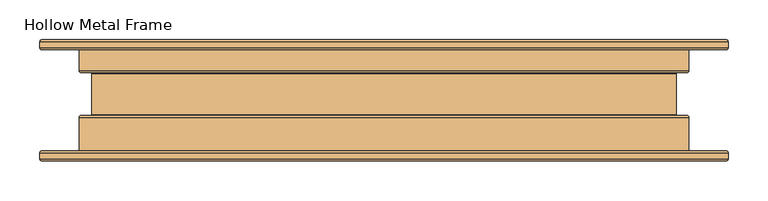
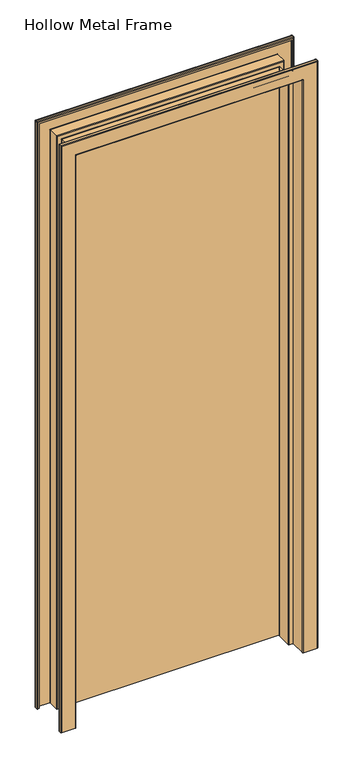
"""IFC4 building model written with IfcOpenShell, lengths in millimetres: door geometry, Hollow Metal Frame."""

from ifc_helpers import new_model, si_unit, frame, origin, origin_with_axes, place, context, project, spatial, polyline, circle_curve, ellipse_curve, outline, extrude, source, transform, mapped, element, save
from ifc_brep_helpers import plane_surface, cylinder_surface, revolved_surface, advanced_brep


def hollow_metal_frame_84e10a40(model_context):
    return source(origin(), model_context, "Body", "SolidModel", [
        advanced_brep(
        [(-429.22825, -63.5635, 0.0), (-423.8625, -63.5635, 0.0), (-423.8625, -65.11925, 0.0), (-429.22825, -65.11925, 0.0), (-430.24425, -66.13525, 0.0), (-430.24425, -73.66, 0.0), (-429.22825, -74.676, 0.0), (-383.57175, -74.676, 0.0), (-382.55575, -73.66, 0.0), (-382.55575, -21.68525, 0.0), (-379.984, -19.1135, 0.0), (-367.69675, -19.1135, 0.0), (-366.68075, -18.0975, 0.0), (-366.68075, 33.6931, 0.0), (-367.69675, 34.7091, 0.0), (-379.984, 34.7091, 0.0), (-382.55575, 37.28085, 0.0), (-382.55575, 73.5965, 0.0), (-383.57175, 74.6125, 0.0), (-429.22825, 74.6125, 0.0), (-430.24425, 73.5965, 0.0), (-430.24425, 66.07175, 0.0), (-429.22825, 65.05575, 0.0), (-423.8625, 65.05575, 0.0), (-423.8625, 63.5, 0.0), (-429.22825, 63.5, 0.0), (-431.8, 66.07175, 0.0), (-431.8, 73.5965, 0.0), (-429.22825, 76.16825, 0.0), (-383.57175, 76.16825, 0.0), (-381.0, 73.5965, 0.0), (-381.0, 37.28085, 0.0), (-379.984, 36.26485, 0.0), (-367.69675, 36.26485, 0.0), (-365.125, 33.6931, 0.0), (-365.125, -18.0975, 0.0), (-367.69675, -20.66925, 0.0), (-379.984, -20.66925, 0.0), (-381.0, -21.68525, 0.0), (-381.0, -73.66, 0.0), (-383.57175, -76.23175, 0.0), (-429.22825, -76.23175, 0.0), (-431.8, -73.66, 0.0), (-431.8, -66.13525, 0.0), (-431.8, -66.13525, 2082.8000001), (-429.22825, -63.5635, 2080.2282501), (-431.8, -73.66, 2082.8000001), (-429.22825, -76.23175, 2080.2282501), (-383.57175, -76.23175, 2034.5717501), (383.57175, -76.23175, 2034.5717501), (383.57175, -76.23175, 0.0), (429.22825, -76.23175, 0.0), (429.22825, -76.23175, 2080.2282501), (-381.0, -73.66, 2032.0000001), (-381.0, -21.68525, 2032.0000001), (-379.984, -20.66925, 2030.9840001), (-367.69675, -20.66925, 2018.6967501), (367.69675, -20.66925, 2018.6967501), (367.69675, -20.66925, 0.0), (379.984, -20.66925, 0.0), (379.984, -20.66925, 2030.9840001), (-365.125, -18.0975, 2016.1250001), (-365.125, 33.6931, 2016.1250001), (-367.69675, 36.26485, 2018.6967501), (-379.984, 36.26485, 2030.9840001), (379.984, 36.26485, 2030.9840001), (379.984, 36.26485, 0.0), (367.69675, 36.26485, 0.0), (367.69675, 36.26485, 2018.6967501), (-381.0, 37.28085, 2032.0000001), (-381.0, 73.5965, 2032.0000001), (-383.57175, 76.16825, 2034.5717501), (-429.22825, 76.16825, 2080.2282501), (429.22825, 76.16825, 2080.2282501), (429.22825, 76.16825, 0.0), (383.57175, 76.16825, 0.0), (383.57175, 76.16825, 2034.5717501), (-431.8, 73.5965, 2082.8000001), (-431.8, 66.07175, 2082.8000001), (-429.22825, 63.5, 2080.2282501), (-423.8625, 63.5, 2074.8625001), (423.8625, 63.5, 2074.8625001), (423.8625, 63.5, 0.0), (429.22825, 63.5, 0.0), (429.22825, 63.5, 2080.2282501), (-423.8625, 65.05575, 2074.8625001), (-429.22825, 65.05575, 2080.2282501), (429.22825, 65.05575, 2080.2282501), (429.22825, 65.05575, 0.0), (423.8625, 65.05575, 0.0), (423.8625, 65.05575, 2074.8625001), (-430.24425, 66.07175, 2081.2442501), (-430.24425, 73.5965, 2081.2442501), (-429.22825, 74.6125, 2080.2282501), (-383.57175, 74.6125, 2034.5717501), (383.57175, 74.6125, 2034.5717501), (383.57175, 74.6125, 0.0), (429.22825, 74.6125, 0.0), (429.22825, 74.6125, 2080.2282501), (-382.55575, 73.5965, 2033.5557501), (-382.55575, 37.28085, 2033.5557501), (-379.984, 34.7091, 2030.9840001), (-367.69675, 34.7091, 2018.6967501), (367.69675, 34.7091, 2018.6967501), (367.69675, 34.7091, 0.0), (379.984, 34.7091, 0.0), (379.984, 34.7091, 2030.9840001), (-366.68075, 33.6931, 2017.6807501), (-366.68075, -18.0975, 2017.6807501), (-367.69675, -19.1135, 2018.6967501), (-379.984, -19.1135, 2030.9840001), (379.984, -19.1135, 2030.9840001), (379.984, -19.1135, 0.0), (367.69675, -19.1135, 0.0), (367.69675, -19.1135, 2018.6967501), (-382.55575, -21.68525, 2033.5557501), (-382.55575, -73.66, 2033.5557501), (-383.57175, -74.676, 2034.5717501), (-429.22825, -74.676, 2080.2282501), (429.22825, -74.676, 2080.2282501), (429.22825, -74.676, 0.0), (383.57175, -74.676, 0.0), (383.57175, -74.676, 2034.5717501), (-430.24425, -73.66, 2081.2442501), (-430.24425, -66.13525, 2081.2442501), (-429.22825, -65.11925, 2080.2282501), (-423.8625, -65.11925, 2074.8625001), (423.8625, -65.11925, 2074.8625001), (423.8625, -65.11925, 0.0), (429.22825, -65.11925, 0.0), (429.22825, -65.11925, 2080.2282501), (-423.8625, -63.5635, 2074.8625001), (429.22825, -63.5635, 2080.2282501), (429.22825, -63.5635, 0.0), (423.8625, -63.5635, 0.0), (423.8625, -63.5635, 2074.8625001), (431.8, -66.13525, 2082.8000001), (431.8, -73.66, 2082.8000001), (381.0, -73.66, 2032.0000001), (381.0, -21.68525, 2032.0000001), (365.125, -18.0975, 2016.1250001), (365.125, 33.6931, 2016.1250001), (381.0, 37.28085, 2032.0000001), (381.0, 73.5965, 2032.0000001), (431.8, 73.5965, 2082.8000001), (431.8, 66.07175, 2082.8000001), (430.24425, 66.07175, 2081.2442501), (430.24425, 73.5965, 2081.2442501), (382.55575, 73.5965, 2033.5557501), (382.55575, 37.28085, 2033.5557501), (366.68075, 33.6931, 2017.6807501), (366.68075, -18.0975, 2017.6807501), (382.55575, -21.68525, 2033.5557501), (382.55575, -73.66, 2033.5557501), (430.24425, -73.66, 2081.2442501), (430.24425, -66.13525, 2081.2442501), (431.8, -66.13525, 0.0), (431.8, -73.66, 0.0), (381.0, -73.66, 0.0), (381.0, -21.68525, 0.0), (365.125, -18.0975, 0.0), (365.125, 33.6931, 0.0), (381.0, 37.28085, 0.0), (381.0, 73.5965, 0.0), (431.8, 73.5965, 0.0), (431.8, 66.07175, 0.0), (430.24425, 66.07175, 0.0), (430.24425, 73.5965, 0.0), (382.55575, 73.5965, 0.0), (382.55575, 37.28085, 0.0), (366.68075, 33.6931, 0.0), (366.68075, -18.0975, 0.0), (382.55575, -21.68525, 0.0), (382.55575, -73.66, 0.0), (430.24425, -73.66, 0.0), (430.24425, -66.13525, 0.0)],
        [
            (0, 1),
            (1, 2),
            (2, 3),
            (3, 4, circle_curve(frame((-429.22825, -66.13525, 0.0), z_axis=(0.0, 0.0, 1.0), x_axis=(0.0, 1.0, 0.0)), 1.016)),
            (4, 5),
            (5, 6, circle_curve(frame((-429.22825, -73.66, 0.0), z_axis=(0.0, 0.0, 1.0), x_axis=(0.0, 1.0, 0.0)), 1.016)),
            (6, 7),
            (7, 8, circle_curve(frame((-383.57175, -73.66, 0.0), z_axis=(0.0, 0.0, 1.0), x_axis=(0.0, 1.0, 0.0)), 1.016)),
            (8, 9),
            (9, 10, circle_curve(frame((-379.984, -21.68525, 0.0), z_axis=(0.0, 0.0, -1.0), x_axis=(0.0, 1.0, 0.0)), 2.57175)),
            (10, 11),
            (11, 12, circle_curve(frame((-367.69675, -18.0975, 0.0), z_axis=(0.0, 0.0, 1.0), x_axis=(0.0, 1.0, 0.0)), 1.016)),
            (12, 13),
            (13, 14, circle_curve(frame((-367.69675, 33.6931, 0.0), z_axis=(0.0, 0.0, 1.0), x_axis=(0.0, 1.0, 0.0)), 1.016)),
            (14, 15),
            (15, 16, circle_curve(frame((-379.984, 37.28085, 0.0), z_axis=(0.0, 0.0, -1.0), x_axis=(0.0, 1.0, 0.0)), 2.57175)),
            (16, 17),
            (17, 18, circle_curve(frame((-383.57175, 73.5965, 0.0), z_axis=(0.0, 0.0, 1.0), x_axis=(0.0, 1.0, 0.0)), 1.016)),
            (18, 19),
            (19, 20, circle_curve(frame((-429.22825, 73.5965, 0.0), z_axis=(0.0, 0.0, 1.0), x_axis=(0.0, 1.0, 0.0)), 1.016)),
            (20, 21),
            (21, 22, circle_curve(frame((-429.22825, 66.07175, 0.0), z_axis=(0.0, 0.0, 1.0), x_axis=(0.0, 1.0, 0.0)), 1.016)),
            (22, 23),
            (23, 24),
            (24, 25),
            (25, 26, circle_curve(frame((-429.22825, 66.07175, 0.0), z_axis=(0.0, 0.0, -1.0), x_axis=(0.0, 1.0, 0.0)), 2.57175)),
            (26, 27),
            (27, 28, circle_curve(frame((-429.22825, 73.5965, 0.0), z_axis=(0.0, 0.0, -1.0), x_axis=(0.0, 1.0, 0.0)), 2.57175)),
            (28, 29),
            (29, 30, circle_curve(frame((-383.57175, 73.5965, 0.0), z_axis=(0.0, 0.0, -1.0), x_axis=(0.0, 1.0, 0.0)), 2.57175)),
            (30, 31),
            (31, 32, circle_curve(frame((-379.984, 37.28085, 0.0), z_axis=(0.0, 0.0, 1.0), x_axis=(0.0, 1.0, 0.0)), 1.016)),
            (32, 33),
            (33, 34, circle_curve(frame((-367.69675, 33.6931, 0.0), z_axis=(0.0, 0.0, -1.0), x_axis=(0.0, 1.0, 0.0)), 2.57175)),
            (34, 35),
            (35, 36, circle_curve(frame((-367.69675, -18.0975, 0.0), z_axis=(0.0, 0.0, -1.0), x_axis=(0.0, 1.0, 0.0)), 2.57175)),
            (36, 37),
            (37, 38, circle_curve(frame((-379.984, -21.68525, 0.0), z_axis=(0.0, 0.0, 1.0), x_axis=(0.0, 1.0, 0.0)), 1.016)),
            (38, 39),
            (39, 40, circle_curve(frame((-383.57175, -73.66, 0.0), z_axis=(0.0, 0.0, -1.0), x_axis=(0.0, 1.0, 0.0)), 2.57175)),
            (40, 41),
            (41, 42, circle_curve(frame((-429.22825, -73.66, 0.0), z_axis=(0.0, 0.0, -1.0), x_axis=(0.0, 1.0, 0.0)), 2.57175)),
            (42, 43),
            (43, 0, circle_curve(frame((-429.22825, -66.13525, 0.0), z_axis=(0.0, 0.0, -1.0), x_axis=(0.0, 1.0, 0.0)), 2.57175)),
            (43, 44),
            (44, 45, ellipse_curve(frame((-429.22825, -66.13525, 2080.2282501), z_axis=(-0.7071067811865475, 0.0, -0.7071067811865475), x_axis=(0.7071067811865474, 0.0, -0.7071067811865476)), 3.6370037, 2.57175)),
            (45, 0),
            (42, 46),
            (46, 44),
            (41, 47),
            (47, 46, ellipse_curve(frame((-429.22825, -73.66, 2080.2282501), z_axis=(-0.7071067811865475, 0.0, -0.7071067811865475), x_axis=(0.7071067811865474, 0.0, -0.7071067811865476)), 3.6370037, 2.57175)),
            (40, 48),
            (48, 49),
            (49, 50),
            (50, 51),
            (51, 52),
            (52, 47),
            (39, 53),
            (53, 48, ellipse_curve(frame((-383.57175, -73.66, 2034.5717501), z_axis=(-0.7071067811865475, 0.0, -0.7071067811865475), x_axis=(0.7071067811865474, 0.0, -0.7071067811865476)), 3.6370037, 2.57175)),
            (38, 54),
            (54, 53),
            (37, 55),
            (55, 54, ellipse_curve(frame((-379.984, -21.68525, 2030.9840001), z_axis=(0.7071067811865475, 0.0, 0.7071067811865475), x_axis=(-0.7071067811865474, 0.0, 0.7071067811865476)), 1.436841, 1.016)),
            (36, 56),
            (56, 57),
            (57, 58),
            (58, 59),
            (59, 60),
            (60, 55),
            (35, 61),
            (61, 56, ellipse_curve(frame((-367.69675, -18.0975, 2018.6967501), z_axis=(-0.7071067811865475, 0.0, -0.7071067811865475), x_axis=(0.7071067811865474, 0.0, -0.7071067811865476)), 3.6370037, 2.57175)),
            (34, 62),
            (62, 61),
            (33, 63),
            (63, 62, ellipse_curve(frame((-367.69675, 33.6931, 2018.6967501), z_axis=(-0.7071067811865475, 0.0, -0.7071067811865475), x_axis=(0.7071067811865474, 0.0, -0.7071067811865476)), 3.6370037, 2.57175)),
            (32, 64),
            (64, 65),
            (65, 66),
            (66, 67),
            (67, 68),
            (68, 63),
            (31, 69),
            (69, 64, ellipse_curve(frame((-379.984, 37.28085, 2030.9840001), z_axis=(0.7071067811865475, 0.0, 0.7071067811865475), x_axis=(-0.7071067811865474, 0.0, 0.7071067811865476)), 1.436841, 1.016)),
            (30, 70),
            (70, 69),
            (29, 71),
            (71, 70, ellipse_curve(frame((-383.57175, 73.5965, 2034.5717501), z_axis=(-0.7071067811865475, 0.0, -0.7071067811865475), x_axis=(0.7071067811865474, 0.0, -0.7071067811865476)), 3.6370037, 2.57175)),
            (28, 72),
            (72, 73),
            (73, 74),
            (74, 75),
            (75, 76),
            (76, 71),
            (27, 77),
            (77, 72, ellipse_curve(frame((-429.22825, 73.5965, 2080.2282501), z_axis=(-0.7071067811865475, 0.0, -0.7071067811865475), x_axis=(0.7071067811865474, 0.0, -0.7071067811865476)), 3.6370037, 2.57175)),
            (26, 78),
            (78, 77),
            (25, 79),
            (79, 78, ellipse_curve(frame((-429.22825, 66.07175, 2080.2282501), z_axis=(-0.7071067811865475, 0.0, -0.7071067811865475), x_axis=(0.7071067811865474, 0.0, -0.7071067811865476)), 3.6370037, 2.57175)),
            (24, 80),
            (80, 81),
            (81, 82),
            (82, 83),
            (83, 84),
            (84, 79),
            (23, 85),
            (85, 80),
            (22, 86),
            (86, 87),
            (87, 88),
            (88, 89),
            (89, 90),
            (90, 85),
            (21, 91),
            (91, 86, ellipse_curve(frame((-429.22825, 66.07175, 2080.2282501), z_axis=(0.7071067811865475, 0.0, 0.7071067811865475), x_axis=(-0.7071067811865474, 0.0, 0.7071067811865476)), 1.436841, 1.016)),
            (20, 92),
            (92, 91),
            (19, 93),
            (93, 92, ellipse_curve(frame((-429.22825, 73.5965, 2080.2282501), z_axis=(0.7071067811865475, 0.0, 0.7071067811865475), x_axis=(-0.7071067811865474, 0.0, 0.7071067811865476)), 1.436841, 1.016)),
            (18, 94),
            (94, 95),
            (95, 96),
            (96, 97),
            (97, 98),
            (98, 93),
            (17, 99),
            (99, 94, ellipse_curve(frame((-383.57175, 73.5965, 2034.5717501), z_axis=(0.7071067811865475, 0.0, 0.7071067811865475), x_axis=(-0.7071067811865474, 0.0, 0.7071067811865476)), 1.436841, 1.016)),
            (16, 100),
            (100, 99),
            (15, 101),
            (101, 100, ellipse_curve(frame((-379.984, 37.28085, 2030.9840001), z_axis=(-0.7071067811865475, 0.0, -0.7071067811865475), x_axis=(0.7071067811865474, 0.0, -0.7071067811865476)), 3.6370037, 2.57175)),
            (14, 102),
            (102, 103),
            (103, 104),
            (104, 105),
            (105, 106),
            (106, 101),
            (13, 107),
            (107, 102, ellipse_curve(frame((-367.69675, 33.6931, 2018.6967501), z_axis=(0.7071067811865475, 0.0, 0.7071067811865475), x_axis=(-0.7071067811865474, 0.0, 0.7071067811865476)), 1.436841, 1.016)),
            (12, 108),
            (108, 107),
            (11, 109),
            (109, 108, ellipse_curve(frame((-367.69675, -18.0975, 2018.6967501), z_axis=(0.7071067811865475, 0.0, 0.7071067811865475), x_axis=(-0.7071067811865474, 0.0, 0.7071067811865476)), 1.436841, 1.016)),
            (10, 110),
            (110, 111),
            (111, 112),
            (112, 113),
            (113, 114),
            (114, 109),
            (9, 115),
            (115, 110, ellipse_curve(frame((-379.984, -21.68525, 2030.9840001), z_axis=(-0.7071067811865475, 0.0, -0.7071067811865475), x_axis=(0.7071067811865474, 0.0, -0.7071067811865476)), 3.6370037, 2.57175)),
            (8, 116),
            (116, 115),
            (7, 117),
            (117, 116, ellipse_curve(frame((-383.57175, -73.66, 2034.5717501), z_axis=(0.7071067811865475, 0.0, 0.7071067811865475), x_axis=(-0.7071067811865474, 0.0, 0.7071067811865476)), 1.436841, 1.016)),
            (6, 118),
            (118, 119),
            (119, 120),
            (120, 121),
            (121, 122),
            (122, 117),
            (5, 123),
            (123, 118, ellipse_curve(frame((-429.22825, -73.66, 2080.2282501), z_axis=(0.7071067811865475, 0.0, 0.7071067811865475), x_axis=(-0.7071067811865474, 0.0, 0.7071067811865476)), 1.436841, 1.016)),
            (4, 124),
            (124, 123),
            (3, 125),
            (125, 124, ellipse_curve(frame((-429.22825, -66.13525, 2080.2282501), z_axis=(0.7071067811865475, 0.0, 0.7071067811865475), x_axis=(-0.7071067811865474, 0.0, 0.7071067811865476)), 1.436841, 1.016)),
            (2, 126),
            (126, 127),
            (127, 128),
            (128, 129),
            (129, 130),
            (130, 125),
            (1, 131),
            (131, 126),
            (45, 132),
            (132, 133),
            (133, 134),
            (134, 135),
            (135, 131),
            (44, 136),
            (136, 132, ellipse_curve(frame((429.22825, -66.13525, 2080.2282501), z_axis=(-0.7071067811865475, 0.0, 0.7071067811865475), x_axis=(-0.7071067811865476, 0.0, -0.7071067811865474)), 3.6370037, 2.57175)),
            (46, 137),
            (137, 136),
            (52, 137, ellipse_curve(frame((429.22825, -73.66, 2080.2282501), z_axis=(-0.7071067811865475, 0.0, 0.7071067811865475), x_axis=(-0.7071067811865476, 0.0, -0.7071067811865474)), 3.6370037, 2.57175)),
            (53, 138),
            (138, 49, ellipse_curve(frame((383.57175, -73.66, 2034.5717501), z_axis=(-0.7071067811865475, 0.0, 0.7071067811865475), x_axis=(-0.7071067811865476, 0.0, -0.7071067811865474)), 3.6370037, 2.57175)),
            (54, 139),
            (139, 138),
            (60, 139, ellipse_curve(frame((379.984, -21.68525, 2030.9840001), z_axis=(0.7071067811865475, 0.0, -0.7071067811865475), x_axis=(0.7071067811865476, 0.0, 0.7071067811865474)), 1.436841, 1.016)),
            (61, 140),
            (140, 57, ellipse_curve(frame((367.69675, -18.0975, 2018.6967501), z_axis=(-0.7071067811865475, 0.0, 0.7071067811865475), x_axis=(-0.7071067811865476, 0.0, -0.7071067811865474)), 3.6370037, 2.57175)),
            (62, 141),
            (141, 140),
            (68, 141, ellipse_curve(frame((367.69675, 33.6931, 2018.6967501), z_axis=(-0.7071067811865475, 0.0, 0.7071067811865475), x_axis=(-0.7071067811865476, 0.0, -0.7071067811865474)), 3.6370037, 2.57175)),
            (69, 142),
            (142, 65, ellipse_curve(frame((379.984, 37.28085, 2030.9840001), z_axis=(0.7071067811865475, 0.0, -0.7071067811865475), x_axis=(0.7071067811865476, 0.0, 0.7071067811865474)), 1.436841, 1.016)),
            (70, 143),
            (143, 142),
            (76, 143, ellipse_curve(frame((383.57175, 73.5965, 2034.5717501), z_axis=(-0.7071067811865475, 0.0, 0.7071067811865475), x_axis=(-0.7071067811865476, 0.0, -0.7071067811865474)), 3.6370037, 2.57175)),
            (77, 144),
            (144, 73, ellipse_curve(frame((429.22825, 73.5965, 2080.2282501), z_axis=(-0.7071067811865475, 0.0, 0.7071067811865475), x_axis=(-0.7071067811865476, 0.0, -0.7071067811865474)), 3.6370037, 2.57175)),
            (78, 145),
            (145, 144),
            (84, 145, ellipse_curve(frame((429.22825, 66.07175, 2080.2282501), z_axis=(-0.7071067811865475, 0.0, 0.7071067811865475), x_axis=(-0.7071067811865476, 0.0, -0.7071067811865474)), 3.6370037, 2.57175)),
            (90, 81),
            (91, 146),
            (146, 87, ellipse_curve(frame((429.22825, 66.07175, 2080.2282501), z_axis=(0.7071067811865475, 0.0, -0.7071067811865475), x_axis=(0.7071067811865476, 0.0, 0.7071067811865474)), 1.436841, 1.016)),
            (92, 147),
            (147, 146),
            (98, 147, ellipse_curve(frame((429.22825, 73.5965, 2080.2282501), z_axis=(0.7071067811865475, 0.0, -0.7071067811865475), x_axis=(0.7071067811865476, 0.0, 0.7071067811865474)), 1.436841, 1.016)),
            (99, 148),
            (148, 95, ellipse_curve(frame((383.57175, 73.5965, 2034.5717501), z_axis=(0.7071067811865475, 0.0, -0.7071067811865475), x_axis=(0.7071067811865476, 0.0, 0.7071067811865474)), 1.436841, 1.016)),
            (100, 149),
            (149, 148),
            (106, 149, ellipse_curve(frame((379.984, 37.28085, 2030.9840001), z_axis=(-0.7071067811865475, 0.0, 0.7071067811865475), x_axis=(-0.7071067811865476, 0.0, -0.7071067811865474)), 3.6370037, 2.57175)),
            (107, 150),
            (150, 103, ellipse_curve(frame((367.69675, 33.6931, 2018.6967501), z_axis=(0.7071067811865475, 0.0, -0.7071067811865475), x_axis=(0.7071067811865476, 0.0, 0.7071067811865474)), 1.436841, 1.016)),
            (108, 151),
            (151, 150),
            (114, 151, ellipse_curve(frame((367.69675, -18.0975, 2018.6967501), z_axis=(0.7071067811865475, 0.0, -0.7071067811865475), x_axis=(0.7071067811865476, 0.0, 0.7071067811865474)), 1.436841, 1.016)),
            (115, 152),
            (152, 111, ellipse_curve(frame((379.984, -21.68525, 2030.9840001), z_axis=(-0.7071067811865475, 0.0, 0.7071067811865475), x_axis=(-0.7071067811865476, 0.0, -0.7071067811865474)), 3.6370037, 2.57175)),
            (116, 153),
            (153, 152),
            (122, 153, ellipse_curve(frame((383.57175, -73.66, 2034.5717501), z_axis=(0.7071067811865475, 0.0, -0.7071067811865475), x_axis=(0.7071067811865476, 0.0, 0.7071067811865474)), 1.436841, 1.016)),
            (123, 154),
            (154, 119, ellipse_curve(frame((429.22825, -73.66, 2080.2282501), z_axis=(0.7071067811865475, 0.0, -0.7071067811865475), x_axis=(0.7071067811865476, 0.0, 0.7071067811865474)), 1.436841, 1.016)),
            (124, 155),
            (155, 154),
            (130, 155, ellipse_curve(frame((429.22825, -66.13525, 2080.2282501), z_axis=(0.7071067811865475, 0.0, -0.7071067811865475), x_axis=(0.7071067811865476, 0.0, 0.7071067811865474)), 1.436841, 1.016)),
            (135, 127),
            (133, 156, circle_curve(frame((429.22825, -66.13525, 0.0), z_axis=(0.0, 0.0, -1.0), x_axis=(0.0, 1.0, 0.0)), 2.57175)),
            (156, 157),
            (157, 51, circle_curve(frame((429.22825, -73.66, 0.0), z_axis=(0.0, 0.0, -1.0), x_axis=(0.0, 1.0, 0.0)), 2.57175)),
            (50, 158, circle_curve(frame((383.57175, -73.66, 0.0), z_axis=(0.0, 0.0, -1.0), x_axis=(0.0, 1.0, 0.0)), 2.57175)),
            (158, 159),
            (159, 59, circle_curve(frame((379.984, -21.68525, 0.0), z_axis=(0.0, 0.0, 1.0), x_axis=(0.0, 1.0, 0.0)), 1.016)),
            (58, 160, circle_curve(frame((367.69675, -18.0975, 0.0), z_axis=(0.0, 0.0, -1.0), x_axis=(0.0, 1.0, 0.0)), 2.57175)),
            (160, 161),
            (161, 67, circle_curve(frame((367.69675, 33.6931, 0.0), z_axis=(0.0, 0.0, -1.0), x_axis=(0.0, 1.0, 0.0)), 2.57175)),
            (66, 162, circle_curve(frame((379.984, 37.28085, 0.0), z_axis=(0.0, 0.0, 1.0), x_axis=(0.0, 1.0, 0.0)), 1.016)),
            (162, 163),
            (163, 75, circle_curve(frame((383.57175, 73.5965, 0.0), z_axis=(0.0, 0.0, -1.0), x_axis=(0.0, 1.0, 0.0)), 2.57175)),
            (74, 164, circle_curve(frame((429.22825, 73.5965, 0.0), z_axis=(0.0, 0.0, -1.0), x_axis=(0.0, 1.0, 0.0)), 2.57175)),
            (164, 165),
            (165, 83, circle_curve(frame((429.22825, 66.07175, 0.0), z_axis=(0.0, 0.0, -1.0), x_axis=(0.0, 1.0, 0.0)), 2.57175)),
            (82, 89),
            (88, 166, circle_curve(frame((429.22825, 66.07175, 0.0), z_axis=(0.0, 0.0, 1.0), x_axis=(0.0, 1.0, 0.0)), 1.016)),
            (166, 167),
            (167, 97, circle_curve(frame((429.22825, 73.5965, 0.0), z_axis=(0.0, 0.0, 1.0), x_axis=(0.0, 1.0, 0.0)), 1.016)),
            (96, 168, circle_curve(frame((383.57175, 73.5965, 0.0), z_axis=(0.0, 0.0, 1.0), x_axis=(0.0, 1.0, 0.0)), 1.016)),
            (168, 169),
            (169, 105, circle_curve(frame((379.984, 37.28085, 0.0), z_axis=(0.0, 0.0, -1.0), x_axis=(0.0, 1.0, 0.0)), 2.57175)),
            (104, 170, circle_curve(frame((367.69675, 33.6931, 0.0), z_axis=(0.0, 0.0, 1.0), x_axis=(0.0, 1.0, 0.0)), 1.016)),
            (170, 171),
            (171, 113, circle_curve(frame((367.69675, -18.0975, 0.0), z_axis=(0.0, 0.0, 1.0), x_axis=(0.0, 1.0, 0.0)), 1.016)),
            (112, 172, circle_curve(frame((379.984, -21.68525, 0.0), z_axis=(0.0, 0.0, -1.0), x_axis=(0.0, 1.0, 0.0)), 2.57175)),
            (172, 173),
            (173, 121, circle_curve(frame((383.57175, -73.66, 0.0), z_axis=(0.0, 0.0, 1.0), x_axis=(0.0, 1.0, 0.0)), 1.016)),
            (120, 174, circle_curve(frame((429.22825, -73.66, 0.0), z_axis=(0.0, 0.0, 1.0), x_axis=(0.0, 1.0, 0.0)), 1.016)),
            (174, 175),
            (175, 129, circle_curve(frame((429.22825, -66.13525, 0.0), z_axis=(0.0, 0.0, 1.0), x_axis=(0.0, 1.0, 0.0)), 1.016)),
            (128, 134),
            (136, 156),
            (137, 157),
            (138, 158),
            (139, 159),
            (140, 160),
            (141, 161),
            (142, 162),
            (143, 163),
            (144, 164),
            (145, 165),
            (146, 166),
            (147, 167),
            (148, 168),
            (149, 169),
            (150, 170),
            (151, 171),
            (152, 172),
            (153, 173),
            (154, 174),
            (155, 175),
        ],
        [
            plane_surface(frame((-392.1125, 63.5, 0.0), z_axis=(0.0, 0.0, -1.0), x_axis=(1.0, 0.0, 0.0))),
            cylinder_surface(frame((-429.22825, -66.13525, 0.0), z_axis=(0.0, 0.0, -1.0), x_axis=(0.0, 1.0, 0.0)), 2.57175),
            plane_surface(frame((-431.8, -66.13525, 0.0), z_axis=(-1.0, 0.0, 0.0), x_axis=(0.0, 0.0, 1.0))),
            cylinder_surface(frame((-429.22825, -73.66, 0.0), z_axis=(0.0, 0.0, -1.0), x_axis=(0.0, 1.0, 0.0)), 2.57175),
            plane_surface(frame((-429.22825, -76.23175, 0.0), z_axis=(0.0, -1.0, 0.0), x_axis=(0.0, 0.0, 1.0))),
            cylinder_surface(frame((-383.57175, -73.66, 0.0), z_axis=(0.0, 0.0, -1.0), x_axis=(0.0, 1.0, 0.0)), 2.57175),
            plane_surface(frame((-381.0, -73.66, 0.0), z_axis=(1.0, 0.0, 0.0), x_axis=(0.0, 0.0, 1.0))),
            revolved_surface(polyline([(-379.984, -20.669249999999998, 2032.0000001145868), (-379.984, -20.669249999999998, 0.0)]), (-379.984, -21.68525, 0.0), (0.0, 0.0, 1.0)),
            plane_surface(frame((-379.984, -20.66925, 0.0), z_axis=(0.0, -1.0, 0.0), x_axis=(0.0, 0.0, 1.0))),
            cylinder_surface(frame((-367.69675, -18.0975, 0.0), z_axis=(0.0, 0.0, -1.0), x_axis=(0.0, 1.0, 0.0)), 2.57175),
            plane_surface(frame((-365.125, -18.0975, 0.0), z_axis=(1.0, 0.0, 0.0), x_axis=(0.0, 0.0, 1.0))),
            cylinder_surface(frame((-367.69675, 33.6931, 0.0), z_axis=(0.0, 0.0, -1.0), x_axis=(0.0, 1.0, 0.0)), 2.57175),
            plane_surface(frame((-367.69675, 36.26485, 0.0), z_axis=(0.0, 1.0, 0.0), x_axis=(0.0, 0.0, 1.0))),
            revolved_surface(polyline([(-379.984, 38.29685, 2032.0000001145868), (-379.984, 38.29685, 0.0)]), (-379.984, 37.28085, 0.0), (0.0, 0.0, 1.0)),
            plane_surface(frame((-381.0, 37.28085, 0.0), z_axis=(1.0, 0.0, 0.0), x_axis=(0.0, 0.0, 1.0))),
            cylinder_surface(frame((-383.57175, 73.5965, 0.0), z_axis=(0.0, 0.0, -1.0), x_axis=(0.0, 1.0, 0.0)), 2.57175),
            plane_surface(frame((-383.57175, 76.16825, 0.0), z_axis=(0.0, 1.0, 0.0), x_axis=(0.0, 0.0, 1.0))),
            cylinder_surface(frame((-429.22825, 73.5965, 0.0), z_axis=(0.0, 0.0, -1.0), x_axis=(0.0, 1.0, 0.0)), 2.57175),
            plane_surface(frame((-431.8, 73.5965, 0.0), z_axis=(-1.0, 0.0, 0.0), x_axis=(0.0, 0.0, 1.0))),
            cylinder_surface(frame((-429.22825, 66.07175, 0.0), z_axis=(0.0, 0.0, -1.0), x_axis=(0.0, 1.0, 0.0)), 2.57175),
            plane_surface(frame((-429.22825, 63.5, 0.0), z_axis=(0.0, -1.0, 0.0), x_axis=(0.0, 0.0, 1.0))),
            plane_surface(frame((-423.8625, 63.5, 0.0), z_axis=(1.0, 0.0, 0.0), x_axis=(0.0, 0.0, 1.0))),
            plane_surface(frame((-423.8625, 65.05575, 0.0), z_axis=(0.0, 1.0, 0.0), x_axis=(0.0, 0.0, 1.0))),
            revolved_surface(polyline([(-429.22825, 67.08775, 2081.244250114587), (-429.22825, 67.08775, 0.0)]), (-429.22825, 66.07175, 0.0), (0.0, 0.0, 1.0)),
            plane_surface(frame((-430.24425, 66.07175, 0.0), z_axis=(1.0, 0.0, 0.0), x_axis=(0.0, 0.0, 1.0))),
            revolved_surface(polyline([(-429.22825, 74.61250000000001, 2081.244250114587), (-429.22825, 74.61250000000001, 0.0)]), (-429.22825, 73.5965, 0.0), (0.0, 0.0, 1.0)),
            plane_surface(frame((-429.22825, 74.6125, 0.0), z_axis=(0.0, -1.0, 0.0), x_axis=(0.0, 0.0, 1.0))),
            revolved_surface(polyline([(-383.57175, 74.61250000000001, 2035.5877501145867), (-383.57175, 74.61250000000001, 0.0)]), (-383.57175, 73.5965, 0.0), (0.0, 0.0, 1.0)),
            plane_surface(frame((-382.55575, 73.5965, 0.0), z_axis=(-1.0, 0.0, 0.0), x_axis=(0.0, 0.0, 1.0))),
            cylinder_surface(frame((-379.984, 37.28085, 0.0), z_axis=(0.0, 0.0, -1.0), x_axis=(0.0, 1.0, 0.0)), 2.57175),
            plane_surface(frame((-379.984, 34.7091, 0.0), z_axis=(0.0, -1.0, 0.0), x_axis=(0.0, 0.0, 1.0))),
            revolved_surface(polyline([(-367.69675, 34.7091, 2019.7127501145867), (-367.69675, 34.7091, 0.0)]), (-367.69675, 33.6931, 0.0), (0.0, 0.0, 1.0)),
            plane_surface(frame((-366.68075, 33.6931, 0.0), z_axis=(-1.0, 0.0, 0.0), x_axis=(0.0, 0.0, 1.0))),
            revolved_surface(polyline([(-367.69675, -17.0815, 2019.7127501145867), (-367.69675, -17.0815, 0.0)]), (-367.69675, -18.0975, 0.0), (0.0, 0.0, 1.0)),
            plane_surface(frame((-367.69675, -19.1135, 0.0), z_axis=(0.0, 1.0, 0.0), x_axis=(0.0, 0.0, 1.0))),
            cylinder_surface(frame((-379.984, -21.68525, 0.0), z_axis=(0.0, 0.0, -1.0), x_axis=(0.0, 1.0, 0.0)), 2.57175),
            plane_surface(frame((-382.55575, -21.68525, 0.0), z_axis=(-1.0, 0.0, 0.0), x_axis=(0.0, 0.0, 1.0))),
            revolved_surface(polyline([(-383.57175, -72.64399999999999, 2035.5877501145867), (-383.57175, -72.64399999999999, 0.0)]), (-383.57175, -73.66, 0.0), (0.0, 0.0, 1.0)),
            plane_surface(frame((-383.57175, -74.676, 0.0), z_axis=(0.0, 1.0, 0.0), x_axis=(0.0, 0.0, 1.0))),
            revolved_surface(polyline([(-429.22825, -72.64399999999999, 2081.244250114587), (-429.22825, -72.64399999999999, 0.0)]), (-429.22825, -73.66, 0.0), (0.0, 0.0, 1.0)),
            plane_surface(frame((-430.24425, -73.66, 0.0), z_axis=(1.0, 0.0, 0.0), x_axis=(0.0, 0.0, 1.0))),
            revolved_surface(polyline([(-429.22825, -65.11925, 2081.244250114587), (-429.22825, -65.11925, 0.0)]), (-429.22825, -66.13525, 0.0), (0.0, 0.0, 1.0)),
            plane_surface(frame((-429.22825, -65.11925, 0.0), z_axis=(0.0, -1.0, 0.0), x_axis=(0.0, 0.0, 1.0))),
            plane_surface(frame((-423.8625, -65.11925, 0.0), z_axis=(1.0, 0.0, 0.0), x_axis=(0.0, 0.0, 1.0))),
            plane_surface(frame((-423.8625, -63.5635, 0.0), z_axis=(0.0, 1.0, 0.0), x_axis=(0.0, 0.0, 1.0))),
            cylinder_surface(frame((-392.1125, -66.13525, 2080.2282501), z_axis=(-1.0, 0.0, 0.0), x_axis=(0.0, 1.0, 0.0)), 2.57175),
            plane_surface(frame((-431.8, -66.13525, 2082.8000001), z_axis=(0.0, 0.0, 1.0), x_axis=(1.0, 0.0, 0.0))),
            cylinder_surface(frame((-392.1125, -73.66, 2080.2282501), z_axis=(-1.0, 0.0, 0.0), x_axis=(0.0, 1.0, 0.0)), 2.57175),
            cylinder_surface(frame((-392.1125, -73.66, 2034.5717501), z_axis=(-1.0, 0.0, 0.0), x_axis=(0.0, 1.0, 0.0)), 2.57175),
            plane_surface(frame((-381.0, -73.66, 2032.0000001), z_axis=(0.0, 0.0, -1.0), x_axis=(1.0, 0.0, 0.0))),
            revolved_surface(polyline([(381.0000000145869, -20.669249999999998, 2030.9840001), (-381.0000000145868, -20.669249999999998, 2030.9840001)]), (-392.1125, -21.68525, 2030.9840001), (1.0, 0.0, 0.0)),
            cylinder_surface(frame((-392.1125, -18.0975, 2018.6967501), z_axis=(-1.0, 0.0, 0.0), x_axis=(0.0, 1.0, 0.0)), 2.57175),
            plane_surface(frame((-365.125, -18.0975, 2016.1250001), z_axis=(0.0, 0.0, -1.0), x_axis=(1.0, 0.0, 0.0))),
            cylinder_surface(frame((-392.1125, 33.6931, 2018.6967501), z_axis=(-1.0, 0.0, 0.0), x_axis=(0.0, 1.0, 0.0)), 2.57175),
            revolved_surface(polyline([(381.0000000145869, 38.29685, 2030.9840001), (-381.0000000145868, 38.29685, 2030.9840001)]), (-392.1125, 37.28085, 2030.9840001), (1.0, 0.0, 0.0)),
            plane_surface(frame((-381.0, 37.28085, 2032.0000001), z_axis=(0.0, 0.0, -1.0), x_axis=(1.0, 0.0, 0.0))),
            cylinder_surface(frame((-392.1125, 73.5965, 2034.5717501), z_axis=(-1.0, 0.0, 0.0), x_axis=(0.0, 1.0, 0.0)), 2.57175),
            cylinder_surface(frame((-392.1125, 73.5965, 2080.2282501), z_axis=(-1.0, 0.0, 0.0), x_axis=(0.0, 1.0, 0.0)), 2.57175),
            plane_surface(frame((-431.8, 73.5965, 2082.8000001), z_axis=(0.0, 0.0, 1.0), x_axis=(1.0, 0.0, 0.0))),
            cylinder_surface(frame((-392.1125, 66.07175, 2080.2282501), z_axis=(-1.0, 0.0, 0.0), x_axis=(0.0, 1.0, 0.0)), 2.57175),
            plane_surface(frame((-423.8625, 63.5, 2074.8625001), z_axis=(0.0, 0.0, -1.0), x_axis=(1.0, 0.0, 0.0))),
            revolved_surface(polyline([(430.24425001458695, 67.08775, 2080.2282501), (-430.24425001458684, 67.08775, 2080.2282501)]), (-392.1125, 66.07175, 2080.2282501), (1.0, 0.0, 0.0)),
            plane_surface(frame((-430.24425, 66.07175, 2081.2442501), z_axis=(0.0, 0.0, -1.0), x_axis=(1.0, 0.0, 0.0))),
            revolved_surface(polyline([(430.24425001458695, 74.61250000000001, 2080.2282501), (-430.24425001458684, 74.61250000000001, 2080.2282501)]), (-392.1125, 73.5965, 2080.2282501), (1.0, 0.0, 0.0)),
            revolved_surface(polyline([(384.5877500145869, 74.61250000000001, 2034.5717501), (-384.58775001458685, 74.61250000000001, 2034.5717501)]), (-392.1125, 73.5965, 2034.5717501), (1.0, 0.0, 0.0)),
            plane_surface(frame((-382.55575, 73.5965, 2033.5557501), z_axis=(0.0, 0.0, 1.0), x_axis=(1.0, 0.0, 0.0))),
            cylinder_surface(frame((-392.1125, 37.28085, 2030.9840001), z_axis=(-1.0, 0.0, 0.0), x_axis=(0.0, 1.0, 0.0)), 2.57175),
            revolved_surface(polyline([(368.7127500145869, 34.7091, 2018.6967501), (-368.71275001458685, 34.7091, 2018.6967501)]), (-392.1125, 33.6931, 2018.6967501), (1.0, 0.0, 0.0)),
            plane_surface(frame((-366.68075, 33.6931, 2017.6807501), z_axis=(0.0, 0.0, 1.0), x_axis=(1.0, 0.0, 0.0))),
            revolved_surface(polyline([(368.7127500145869, -17.0815, 2018.6967501), (-368.71275001458685, -17.0815, 2018.6967501)]), (-392.1125, -18.0975, 2018.6967501), (1.0, 0.0, 0.0)),
            cylinder_surface(frame((-392.1125, -21.68525, 2030.9840001), z_axis=(-1.0, 0.0, 0.0), x_axis=(0.0, 1.0, 0.0)), 2.57175),
            plane_surface(frame((-382.55575, -21.68525, 2033.5557501), z_axis=(0.0, 0.0, 1.0), x_axis=(1.0, 0.0, 0.0))),
            revolved_surface(polyline([(384.5877500145869, -72.64399999999999, 2034.5717501), (-384.58775001458685, -72.64399999999999, 2034.5717501)]), (-392.1125, -73.66, 2034.5717501), (1.0, 0.0, 0.0)),
            revolved_surface(polyline([(430.24425001458695, -72.64399999999999, 2080.2282501), (-430.24425001458684, -72.64399999999999, 2080.2282501)]), (-392.1125, -73.66, 2080.2282501), (1.0, 0.0, 0.0)),
            plane_surface(frame((-430.24425, -73.66, 2081.2442501), z_axis=(0.0, 0.0, -1.0), x_axis=(1.0, 0.0, 0.0))),
            revolved_surface(polyline([(430.24425001458695, -65.11925, 2080.2282501), (-430.24425001458684, -65.11925, 2080.2282501)]), (-392.1125, -66.13525, 2080.2282501), (1.0, 0.0, 0.0)),
            plane_surface(frame((-423.8625, -65.11925, 2074.8625001), z_axis=(0.0, 0.0, -1.0), x_axis=(1.0, 0.0, 0.0))),
            plane_surface(frame((392.1125, 63.5, 0.0), z_axis=(0.0, 0.0, -1.0), x_axis=(-1.0, 0.0, 0.0))),
            cylinder_surface(frame((429.22825, -66.13525, 2043.1125001), z_axis=(0.0, 0.0, 1.0), x_axis=(0.0, 1.0, 0.0)), 2.57175),
            plane_surface(frame((431.8, -66.13525, 2082.8000001), z_axis=(1.0, 0.0, 0.0), x_axis=(0.0, 0.0, -1.0))),
            cylinder_surface(frame((429.22825, -73.66, 2043.1125001), z_axis=(0.0, 0.0, 1.0), x_axis=(0.0, 1.0, 0.0)), 2.57175),
            cylinder_surface(frame((383.57175, -73.66, 2043.1125001), z_axis=(0.0, 0.0, 1.0), x_axis=(0.0, 1.0, 0.0)), 2.57175),
            plane_surface(frame((381.0, -73.66, 2032.0000001), z_axis=(-1.0, 0.0, 0.0), x_axis=(0.0, 0.0, -1.0))),
            revolved_surface(polyline([(379.984, -20.669249999999998, 0.0), (379.984, -20.669249999999998, 2032.0000001145868)]), (379.984, -21.68525, 2043.1125001), (0.0, 0.0, -1.0)),
            cylinder_surface(frame((367.69675, -18.0975, 2043.1125001), z_axis=(0.0, 0.0, 1.0), x_axis=(0.0, 1.0, 0.0)), 2.57175),
            plane_surface(frame((365.125, -18.0975, 2016.1250001), z_axis=(-1.0, 0.0, 0.0), x_axis=(0.0, 0.0, -1.0))),
            cylinder_surface(frame((367.69675, 33.6931, 2043.1125001), z_axis=(0.0, 0.0, 1.0), x_axis=(0.0, 1.0, 0.0)), 2.57175),
            revolved_surface(polyline([(379.984, 38.29685, 0.0), (379.984, 38.29685, 2032.0000001145868)]), (379.984, 37.28085, 2043.1125001), (0.0, 0.0, -1.0)),
            plane_surface(frame((381.0, 37.28085, 2032.0000001), z_axis=(-1.0, 0.0, 0.0), x_axis=(0.0, 0.0, -1.0))),
            cylinder_surface(frame((383.57175, 73.5965, 2043.1125001), z_axis=(0.0, 0.0, 1.0), x_axis=(0.0, 1.0, 0.0)), 2.57175),
            cylinder_surface(frame((429.22825, 73.5965, 2043.1125001), z_axis=(0.0, 0.0, 1.0), x_axis=(0.0, 1.0, 0.0)), 2.57175),
            plane_surface(frame((431.8, 73.5965, 2082.8000001), z_axis=(1.0, 0.0, 0.0), x_axis=(0.0, 0.0, -1.0))),
            cylinder_surface(frame((429.22825, 66.07175, 2043.1125001), z_axis=(0.0, 0.0, 1.0), x_axis=(0.0, 1.0, 0.0)), 2.57175),
            plane_surface(frame((423.8625, 63.5, 2074.8625001), z_axis=(-1.0, 0.0, 0.0), x_axis=(0.0, 0.0, -1.0))),
            revolved_surface(polyline([(429.22825, 67.08775, 0.0), (429.22825, 67.08775, 2081.244250114587)]), (429.22825, 66.07175, 2043.1125001), (0.0, 0.0, -1.0)),
            plane_surface(frame((430.24425, 66.07175, 2081.2442501), z_axis=(-1.0, 0.0, 0.0), x_axis=(0.0, 0.0, -1.0))),
            revolved_surface(polyline([(429.22825, 74.61250000000001, 0.0), (429.22825, 74.61250000000001, 2081.244250114587)]), (429.22825, 73.5965, 2043.1125001), (0.0, 0.0, -1.0)),
            revolved_surface(polyline([(383.57175, 74.61250000000001, 0.0), (383.57175, 74.61250000000001, 2035.5877501145867)]), (383.57175, 73.5965, 2043.1125001), (0.0, 0.0, -1.0)),
            plane_surface(frame((382.55575, 73.5965, 2033.5557501), z_axis=(1.0, 0.0, 0.0), x_axis=(0.0, 0.0, -1.0))),
            cylinder_surface(frame((379.984, 37.28085, 2043.1125001), z_axis=(0.0, 0.0, 1.0), x_axis=(0.0, 1.0, 0.0)), 2.57175),
            revolved_surface(polyline([(367.69675, 34.7091, 0.0), (367.69675, 34.7091, 2019.7127501145867)]), (367.69675, 33.6931, 2043.1125001), (0.0, 0.0, -1.0)),
            plane_surface(frame((366.68075, 33.6931, 2017.6807501), z_axis=(1.0, 0.0, 0.0), x_axis=(0.0, 0.0, -1.0))),
            revolved_surface(polyline([(367.69675, -17.0815, 0.0), (367.69675, -17.0815, 2019.7127501145867)]), (367.69675, -18.0975, 2043.1125001), (0.0, 0.0, -1.0)),
            cylinder_surface(frame((379.984, -21.68525, 2043.1125001), z_axis=(0.0, 0.0, 1.0), x_axis=(0.0, 1.0, 0.0)), 2.57175),
            plane_surface(frame((382.55575, -21.68525, 2033.5557501), z_axis=(1.0, 0.0, 0.0), x_axis=(0.0, 0.0, -1.0))),
            revolved_surface(polyline([(383.57175, -72.64399999999999, 0.0), (383.57175, -72.64399999999999, 2035.5877501145867)]), (383.57175, -73.66, 2043.1125001), (0.0, 0.0, -1.0)),
            revolved_surface(polyline([(429.22825, -72.64399999999999, 0.0), (429.22825, -72.64399999999999, 2081.244250114587)]), (429.22825, -73.66, 2043.1125001), (0.0, 0.0, -1.0)),
            plane_surface(frame((430.24425, -73.66, 2081.2442501), z_axis=(-1.0, 0.0, 0.0), x_axis=(0.0, 0.0, -1.0))),
            revolved_surface(polyline([(429.22825, -65.11925, 0.0), (429.22825, -65.11925, 2081.244250114587)]), (429.22825, -66.13525, 2043.1125001), (0.0, 0.0, -1.0)),
            plane_surface(frame((423.8625, -65.11925, 2074.8625001), z_axis=(-1.0, 0.0, 0.0), x_axis=(0.0, 0.0, -1.0))),
        ],
        [
            (0, [[1, 2, 3, 4, 5, 6, 7, 8, 9, 10, 11, 12, 13, 14, 15, 16, 17, 18, 19, 20, 21, 22, 23, 24, 25, 26, 27, 28, 29, 30, 31, 32, 33, 34, 35, 36, 37, 38, 39, 40, 41, 42, 43, 44]]),
            (1, [[45, 46, 47, -44]]),
            (2, [[48, 49, -45, -43]]),
            (3, [[50, 51, -48, -42]]),
            (4, [[52, 53, 54, 55, 56, 57, -50, -41]]),
            (5, [[58, 59, -52, -40]]),
            (6, [[60, 61, -58, -39]]),
            (7, [[62, 63, -60, -38]]),
            (8, [[64, 65, 66, 67, 68, 69, -62, -37]]),
            (9, [[70, 71, -64, -36]]),
            (10, [[72, 73, -70, -35]]),
            (11, [[74, 75, -72, -34]]),
            (12, [[76, 77, 78, 79, 80, 81, -74, -33]]),
            (13, [[82, 83, -76, -32]]),
            (14, [[84, 85, -82, -31]]),
            (15, [[86, 87, -84, -30]]),
            (16, [[88, 89, 90, 91, 92, 93, -86, -29]]),
            (17, [[94, 95, -88, -28]]),
            (18, [[96, 97, -94, -27]]),
            (19, [[98, 99, -96, -26]]),
            (20, [[100, 101, 102, 103, 104, 105, -98, -25]]),
            (21, [[106, 107, -100, -24]]),
            (22, [[108, 109, 110, 111, 112, 113, -106, -23]]),
            (23, [[114, 115, -108, -22]]),
            (24, [[116, 117, -114, -21]]),
            (25, [[118, 119, -116, -20]]),
            (26, [[120, 121, 122, 123, 124, 125, -118, -19]]),
            (27, [[126, 127, -120, -18]]),
            (28, [[128, 129, -126, -17]]),
            (29, [[130, 131, -128, -16]]),
            (30, [[132, 133, 134, 135, 136, 137, -130, -15]]),
            (31, [[138, 139, -132, -14]]),
            (32, [[140, 141, -138, -13]]),
            (33, [[142, 143, -140, -12]]),
            (34, [[144, 145, 146, 147, 148, 149, -142, -11]]),
            (35, [[150, 151, -144, -10]]),
            (36, [[152, 153, -150, -9]]),
            (37, [[154, 155, -152, -8]]),
            (38, [[156, 157, 158, 159, 160, 161, -154, -7]]),
            (39, [[162, 163, -156, -6]]),
            (40, [[164, 165, -162, -5]]),
            (41, [[166, 167, -164, -4]]),
            (42, [[168, 169, 170, 171, 172, 173, -166, -3]]),
            (43, [[174, 175, -168, -2]]),
            (44, [[-47, 176, 177, 178, 179, 180, -174, -1]]),
            (45, [[181, 182, -176, -46]]),
            (46, [[183, 184, -181, -49]]),
            (47, [[-57, 185, -183, -51]]),
            (48, [[186, 187, -53, -59]]),
            (49, [[188, 189, -186, -61]]),
            (50, [[-69, 190, -188, -63]]),
            (51, [[191, 192, -65, -71]]),
            (52, [[193, 194, -191, -73]]),
            (53, [[-81, 195, -193, -75]]),
            (54, [[196, 197, -77, -83]]),
            (55, [[198, 199, -196, -85]]),
            (56, [[-93, 200, -198, -87]]),
            (57, [[201, 202, -89, -95]]),
            (58, [[203, 204, -201, -97]]),
            (59, [[-105, 205, -203, -99]]),
            (60, [[-113, 206, -101, -107]]),
            (61, [[207, 208, -109, -115]]),
            (62, [[209, 210, -207, -117]]),
            (63, [[-125, 211, -209, -119]]),
            (64, [[212, 213, -121, -127]]),
            (65, [[214, 215, -212, -129]]),
            (66, [[-137, 216, -214, -131]]),
            (67, [[217, 218, -133, -139]]),
            (68, [[219, 220, -217, -141]]),
            (69, [[-149, 221, -219, -143]]),
            (70, [[222, 223, -145, -151]]),
            (71, [[224, 225, -222, -153]]),
            (72, [[-161, 226, -224, -155]]),
            (73, [[227, 228, -157, -163]]),
            (74, [[229, 230, -227, -165]]),
            (75, [[-173, 231, -229, -167]]),
            (76, [[-180, 232, -169, -175]]),
            (77, [[233, 234, 235, -55, 236, 237, 238, -67, 239, 240, 241, -79, 242, 243, 244, -91, 245, 246, 247, -103, 248, -111, 249, 250, 251, -123, 252, 253, 254, -135, 255, 256, 257, -147, 258, 259, 260, -159, 261, 262, 263, -171, 264, -178]]),
            (78, [[265, -233, -177, -182]]),
            (79, [[266, -234, -265, -184]]),
            (80, [[-56, -235, -266, -185]]),
            (81, [[267, -236, -54, -187]]),
            (82, [[268, -237, -267, -189]]),
            (83, [[-68, -238, -268, -190]]),
            (84, [[269, -239, -66, -192]]),
            (85, [[270, -240, -269, -194]]),
            (86, [[-80, -241, -270, -195]]),
            (87, [[271, -242, -78, -197]]),
            (88, [[272, -243, -271, -199]]),
            (89, [[-92, -244, -272, -200]]),
            (90, [[273, -245, -90, -202]]),
            (91, [[274, -246, -273, -204]]),
            (92, [[-104, -247, -274, -205]]),
            (93, [[-112, -248, -102, -206]]),
            (94, [[275, -249, -110, -208]]),
            (95, [[276, -250, -275, -210]]),
            (96, [[-124, -251, -276, -211]]),
            (97, [[277, -252, -122, -213]]),
            (98, [[278, -253, -277, -215]]),
            (99, [[-136, -254, -278, -216]]),
            (100, [[279, -255, -134, -218]]),
            (101, [[280, -256, -279, -220]]),
            (102, [[-148, -257, -280, -221]]),
            (103, [[281, -258, -146, -223]]),
            (104, [[282, -259, -281, -225]]),
            (105, [[-160, -260, -282, -226]]),
            (106, [[283, -261, -158, -228]]),
            (107, [[284, -262, -283, -230]]),
            (108, [[-172, -263, -284, -231]]),
            (109, [[-179, -264, -170, -232]]),
        ],
    ),
        extrude(outline(polyline([(379.44425, 37.28085), (-379.44425, 37.28085), (-379.44425, 63.5), (379.44425, 63.5), (379.44425, 37.28085)])), origin_with_axes(), (0.0, 0.0, 1.0), 2032.0000001),
    ])


if __name__ == "__main__":
    model = new_model("IFC4")
    model_context = context("Model", 3, world=origin())
    ifc_project = project(units=[si_unit("LENGTHUNIT", "METRE", prefix="MILLI")], contexts=[model_context])
    site = spatial("IfcSite", under=ifc_project)
    building = spatial("IfcBuilding", under=site)
    placement = place(None, origin())
    hollow_metal_frame_shape = hollow_metal_frame_84e10a40(model_context)
    element("IfcDoor", 1, ObjectType="Hollow Metal Frame : 2'-6\"W x 6'-8\"H", at=placement, inside=building, context=model_context, shape_type="MappedRepresentation", body=[
        mapped(hollow_metal_frame_shape, transform((0.0, 0.0, 0.0), x_axis=(1.0, 0.0, 0.0), y_axis=(0.0, 1.0, 0.0), z_axis=(0.0, 0.0, 1.0))),
    ])
    save(model, "model.ifc")

# Revit data of these elements
# Type "Hollow Metal Frame : 2'-6\"W x 6'-8\"H"
#   Type Mark = "p"
#   Product Page URL = ""
#   Product Name = ""
#   Product Documentation Link = ""
#   Material = ""
#   DS_Hardware_Set_(SFT) = ""
#   DS_Frame_Type_(SFT) = ""
#   DS_Fire_Rating_(SFT) = ""
#   DS_Door_Type_(SFT) = ""
#   Analytic Construction = "<None>"
#   Frame Projection Ext. = 0' - 1"
#   Frame Projection Int. = 0' - 1"
#   Frame Width = 0' - 3"
#   Height = 6' - 8"
#   Width = 2' - 6"
#   Non-Kerfed = yes
#   Kerfed = no
#   Hollow Metal Casing = Metal-Dunbarton_Doors-White
#   Flush Door = Metal-Dunbarton_Doors-Aluminum
#   DS_Frame_Material_(SFT) = none
#   DS_Door_Material_(SFT) = none
#   URL = ""
#   Model = ""
#   Manufacturer = ""
#   Function = (empty or 0)
#   Wall Closure = (empty or 0)
#   Description = (empty or 0)
# Element 1 (IfcDoor, "Hollow Metal Frame : 2'-6\"W x 6'-8\"H")
#   Materials on its faces: "Metal-Dunbarton_Doors-White", "Metal-Dunbarton_Doors-Aluminum"
# Materials
#   "Metal-Dunbarton_Doors-White": class "Miscellaneous", colour RGB 230 233 236, transparency 0
#   "Metal-Dunbarton_Doors-Aluminum": class "System", colour RGB 143 142 141, transparency 0
